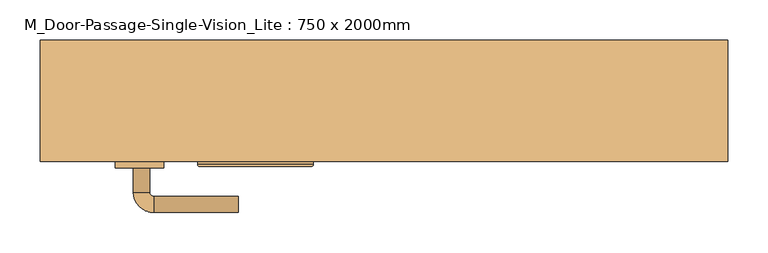
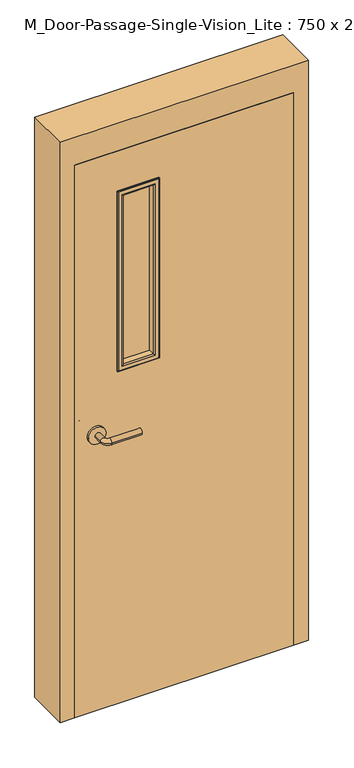
"""IFC4 building model written with IfcOpenShell, lengths in millimetres: door geometry, M_Door-Passage-Single-Vision_Lite : 750 x 2000mm."""

from ifc_helpers import new_model, si_unit, point, frame, frame_2d, origin, place, context, project, spatial, polyline, circle_curve, ellipse_curve, trimmed, segment, composite_curve, outline, extrude, faceted_brep, source, transform, mapped, element, save
from ifc_brep_helpers import plane_surface, cylinder_surface, revolved_surface, advanced_brep


def m_door_passage_single_vision_lite_750_x_2000mm_ab727fbf(model_context):
    return source(origin(), model_context, "Body", "SolidModel", [
        advanced_brep(
        [(-309.990625, 9.15, 1000.0), (-289.990625, 9.15, 1000.0), (-309.990625, 39.15, 1000.0), (-289.990625, 39.15, 1000.0), (-284.990625, 44.15, 1000.0), (-284.990625, 64.15, 1000.0), (-179.990625, 64.15, 1000.0), (-179.990625, 44.15, 1000.0)],
        [
            (0, 1, circle_curve(frame((-299.990625, 9.15, 1000.0), z_axis=(0.0, -1.0, 0.0), x_axis=(1.0, 0.0, 0.0)), 10.0)),
            (1, 0, circle_curve(frame((-299.990625, 9.15, 1000.0), z_axis=(0.0, -1.0, 0.0), x_axis=(1.0, 0.0, 0.0)), 10.0)),
            (0, 2),
            (2, 3, circle_curve(frame((-299.990625, 39.15, 1000.0), z_axis=(0.0, -1.0, 0.0), x_axis=(1.0, 0.0, 0.0)), 10.0)),
            (3, 1),
            (3, 2, circle_curve(frame((-299.990625, 39.15, 1000.0), z_axis=(0.0, -1.0, 0.0), x_axis=(1.0, 0.0, 0.0)), 10.0)),
            (4, 3, circle_curve(frame((-284.990625, 39.15, 1000.0), z_axis=(0.0, 0.0, 1.0), x_axis=(-1.0, 0.0, 0.0)), 5.0)),
            (2, 5, circle_curve(frame((-284.990625, 39.15, 1000.0), z_axis=(0.0, 0.0, -1.0), x_axis=(-1.0, 0.0, 0.0)), 25.0)),
            (5, 4, circle_curve(frame((-284.990625, 54.15, 1000.0), z_axis=(-1.0, 0.0, 0.0), x_axis=(0.0, -1.0, 0.0)), 10.0)),
            (4, 5, circle_curve(frame((-284.990625, 54.15, 1000.0), z_axis=(-1.0, 0.0, 0.0), x_axis=(0.0, -1.0, 0.0)), 10.0)),
            (6, 7, circle_curve(frame((-179.990625, 54.15, 1000.0), z_axis=(1.0, 0.0, 0.0), x_axis=(0.0, -1.0, 0.0)), 10.0)),
            (7, 6, circle_curve(frame((-179.990625, 54.15, 1000.0), z_axis=(1.0, 0.0, 0.0), x_axis=(0.0, -1.0, 0.0)), 10.0)),
            (5, 6),
            (7, 4),
        ],
        [
            plane_surface(frame((-299.990625, 9.15, 1000.0), z_axis=(0.0, -1.0, 0.0), x_axis=(0.0, 0.0, 1.0))),
            cylinder_surface(frame((-299.990625, 9.15, 1000.0), z_axis=(0.0, -1.0, 0.0), x_axis=(1.0, 0.0, 0.0)), 10.0),
            revolved_surface(trimmed(ellipse_curve(frame((-299.990625, 39.15, 1000.0), z_axis=(0.0, -1.0, 0.0), x_axis=(1.0, 0.0, 0.0)), 10.0, 10.0), [point((-309.990625, 39.15, 1000.0))], [point((-289.990625, 39.15, 1000.0))], True, "CARTESIAN"), (-284.990625, 39.15, 1000.0), (0.0, 0.0, -1.0)),
            revolved_surface(trimmed(ellipse_curve(frame((-299.990625, 39.15, 1000.0), z_axis=(0.0, -1.0, 0.0), x_axis=(1.0, 0.0, 0.0)), 10.0, 10.0), [point((-289.990625, 39.15, 1000.0))], [point((-309.990625, 39.15, 1000.0))], True, "CARTESIAN"), (-284.990625, 39.15, 1000.0), (0.0, 0.0, -1.0)),
            plane_surface(frame((-179.990625, 54.15, 1000.0), z_axis=(1.0, 0.0, 0.0), x_axis=(0.0, 0.0, 1.0))),
            cylinder_surface(frame((-284.990625, 54.15, 1000.0), z_axis=(-1.0, 0.0, 0.0), x_axis=(0.0, -1.0, 0.0)), 10.0),
        ],
        [
            (0, [[1, 2]]),
            (1, [[-1, 3, 4, 5]]),
            (1, [[-2, -5, 6, -3]]),
            (2, [[7, -4, 8, 9]]),
            (3, [[-8, -6, -7, 10]]),
            (4, [[11, 12]]),
            (5, [[-9, 13, -12, 14]]),
            (5, [[-10, -14, -11, -13]]),
        ],
    ),
        extrude(outline(composite_curve([segment(trimmed(circle_curve(frame_2d((1000.0, -302.490625)), 30.0), [point((1000.0, -332.490625))], [point((1000.0, -272.490625))], False, "CARTESIAN"), True, "CONTINUOUS"), segment(trimmed(circle_curve(frame_2d((1000.0, -302.490625)), 30.0), [point((1000.0, -272.490625))], [point((1000.0, -332.490625))], False, "CARTESIAN"), True, "CONTINUOUS")], self_intersect=False)), frame((0.0, 1.15, 0.0), z_axis=(0.0, 1.0, 0.0), x_axis=(0.0, 0.0, 1.0)), (0.0, 0.0, 1.0), 8.0),
        advanced_brep(
        [(-309.990625, -51.85, 1000.0), (-289.990625, -51.85, 1000.0), (-289.990625, -81.85, 1000.0), (-309.990625, -81.85, 1000.0), (-284.990625, -86.85, 1000.0), (-284.990625, -106.85, 1000.0), (-179.990625, -106.85, 1000.0), (-179.990625, -86.85, 1000.0)],
        [
            (0, 1, circle_curve(frame((-299.990625, -51.85, 1000.0), z_axis=(0.0, 1.0, 0.0), x_axis=(1.0, 0.0, 0.0)), 10.0)),
            (1, 0, circle_curve(frame((-299.990625, -51.85, 1000.0), z_axis=(0.0, 1.0, 0.0), x_axis=(1.0, 0.0, 0.0)), 10.0)),
            (1, 2),
            (2, 3, circle_curve(frame((-299.990625, -81.85, 1000.0), z_axis=(0.0, 1.0, 0.0), x_axis=(1.0, 0.0, 0.0)), 10.0)),
            (3, 0),
            (3, 2, circle_curve(frame((-299.990625, -81.85, 1000.0), z_axis=(0.0, 1.0, 0.0), x_axis=(1.0, 0.0, 0.0)), 10.0)),
            (4, 5, circle_curve(frame((-284.990625, -96.85, 1000.0), z_axis=(-1.0, 0.0, 0.0), x_axis=(0.0, 1.0, 0.0)), 10.0)),
            (5, 3, circle_curve(frame((-284.990625, -81.85, 1000.0), z_axis=(0.0, 0.0, -1.0), x_axis=(-1.0, 0.0, 0.0)), 25.0)),
            (2, 4, circle_curve(frame((-284.990625, -81.85, 1000.0), z_axis=(0.0, 0.0, 1.0), x_axis=(-1.0, 0.0, 0.0)), 5.0)),
            (5, 4, circle_curve(frame((-284.990625, -96.85, 1000.0), z_axis=(-1.0, 0.0, 0.0), x_axis=(0.0, 1.0, 0.0)), 10.0)),
            (6, 7, circle_curve(frame((-179.990625, -96.85, 1000.0), z_axis=(1.0, 0.0, 0.0), x_axis=(0.0, 1.0, 0.0)), 10.0)),
            (7, 6, circle_curve(frame((-179.990625, -96.85, 1000.0), z_axis=(1.0, 0.0, 0.0), x_axis=(0.0, 1.0, 0.0)), 10.0)),
            (4, 7),
            (6, 5),
        ],
        [
            plane_surface(frame((-299.990625, -51.85, 1000.0), z_axis=(0.0, 1.0, 0.0), x_axis=(0.0, 0.0, 1.0))),
            cylinder_surface(frame((-299.990625, -51.85, 1000.0), z_axis=(0.0, 1.0, 0.0), x_axis=(1.0, 0.0, 0.0)), 10.0),
            revolved_surface(trimmed(ellipse_curve(frame((-299.990625, -81.85, 1000.0), z_axis=(0.0, -1.0, 0.0), x_axis=(1.0, 0.0, 0.0)), 10.0, 10.0), [point((-309.990625, -81.85, 1000.0))], [point((-289.990625, -81.85, 1000.0))], True, "CARTESIAN"), (-284.990625, -81.85, 1000.0), (0.0, 0.0, -1.0)),
            revolved_surface(trimmed(ellipse_curve(frame((-299.990625, -81.85, 1000.0), z_axis=(0.0, -1.0, 0.0), x_axis=(1.0, 0.0, 0.0)), 10.0, 10.0), [point((-289.990625, -81.85, 1000.0))], [point((-309.990625, -81.85, 1000.0))], True, "CARTESIAN"), (-284.990625, -81.85, 1000.0), (0.0, 0.0, -1.0)),
            plane_surface(frame((-179.990625, -96.85, 1000.0), z_axis=(1.0, 0.0, 0.0), x_axis=(0.0, 0.0, 1.0))),
            cylinder_surface(frame((-284.990625, -96.85, 1000.0), z_axis=(-1.0, 0.0, 0.0), x_axis=(0.0, 1.0, 0.0)), 10.0),
        ],
        [
            (0, [[1, 2]]),
            (1, [[3, 4, 5, -2]]),
            (1, [[-5, 6, -3, -1]]),
            (2, [[7, 8, -4, 9]]),
            (3, [[10, -9, -6, -8]]),
            (4, [[11, 12]]),
            (5, [[13, -11, 14, -7]]),
            (5, [[-14, -12, -13, -10]]),
        ],
    ),
        extrude(outline(composite_curve([segment(trimmed(circle_curve(frame_2d((1000.0, -302.490625)), 30.0), [point((1000.0, -332.490625))], [point((1000.0, -272.490625))], False, "CARTESIAN"), True, "CONTINUOUS"), segment(trimmed(circle_curve(frame_2d((1000.0, -302.490625)), 30.0), [point((1000.0, -272.490625))], [point((1000.0, -332.490625))], False, "CARTESIAN"), True, "CONTINUOUS")], self_intersect=False)), frame((0.0, -51.85, 0.0), z_axis=(0.0, 1.0, 0.0), x_axis=(0.0, 0.0, 1.0)), (0.0, 0.0, 1.0), 8.0),
        extrude(outline(polyline([(2000.0, -375.0), (0.0, -375.0), (0.0, 375.0), (2000.0, 375.0), (2000.0, -375.0)]), holes=[polyline([(1847.6, -222.6), (1847.6, -95.6), (1212.6, -95.6), (1212.6, -222.6), (1847.6, -222.6)])]), frame((0.0, -43.85, 0.0), z_axis=(0.0, 1.0, 0.0), x_axis=(0.0, 0.0, 1.0)), (0.0, 0.0, 1.0), 45.0),
        faceted_brep([(375.0, 5.9125, 0.0), (359.125, 5.9125, 0.0), (359.125, 56.9375, 0.0), (375.0, 56.9375, 0.0), (375.0, 106.15, 0.0), (425.0, 106.15, 0.0), (425.0, -43.85, 0.0), (375.0, -43.85, 0.0), (375.0, -43.85, 2000.0), (375.0, 5.9125, 2000.0), (425.0, -43.85, 2100.0), (-425.0, -43.85, 2100.0), (-425.0, -43.85, 0.0), (-375.0, -43.85, 0.0), (-375.0, -43.85, 2000.0), (425.0, 106.15, 2100.0), (375.0, 106.15, 2000.0), (-375.0, 106.15, 2000.0), (-375.0, 106.15, 0.0), (-425.0, 106.15, 0.0), (-425.0, 106.15, 2100.0), (375.0, 56.9375, 2000.0), (359.125, 56.9375, 1984.125), (-359.125, 56.9375, 1984.125), (-359.125, 56.9375, 0.0), (-375.0, 56.9375, 0.0), (-375.0, 56.9375, 2000.0), (359.125, 5.9125, 1984.125), (-375.0, 5.9125, 2000.0), (-375.0, 5.9125, 0.0), (-359.125, 5.9125, 0.0), (-359.125, 5.9125, 1984.125)], [[[0, 1, 2, 3, 4, 5, 6, 7]], [[7, 8, 9, 0]], [[6, 10, 11, 12, 13, 14, 8, 7]], [[5, 15, 10, 6]], [[4, 16, 17, 18, 19, 20, 15, 5]], [[3, 21, 16, 4]], [[2, 22, 23, 24, 25, 26, 21, 3]], [[1, 27, 22, 2]], [[0, 9, 28, 29, 30, 31, 27, 1]], [[8, 14, 28, 9]], [[16, 21, 26, 17]], [[22, 27, 31, 23]], [[12, 19, 18, 25, 24, 30, 29, 13]], [[13, 29, 28, 14]], [[11, 20, 19, 12]], [[17, 26, 25, 18]], [[23, 31, 30, 24]], [[15, 20, 11, 10]]]),
        extrude(outline(polyline([(-95.6, -18.85), (-95.6, -23.85), (-222.6, -23.85), (-222.6, -18.85), (-95.6, -18.85)])), frame((0.0, 0.0, 1212.6), z_axis=(0.0, 0.0, 1.0), x_axis=(1.0, 0.0, 0.0)), (0.0, 0.0, 1.0), 635.0),
        advanced_brep(
        [(-222.6, -23.85, 1847.6), (-222.6, -23.85, 1212.6), (-222.6, -43.85, 1212.6), (-222.6, -43.85, 1847.6), (-210.6, -44.85, 1835.6), (-210.6, -44.85, 1224.6), (-210.6, -23.85, 1224.6), (-210.6, -23.85, 1835.6), (-215.6, -49.85, 1840.6), (-215.6, -49.85, 1219.6), (-230.6, -47.85, 1855.6), (-230.6, -47.85, 1204.6), (-228.6, -49.85, 1206.6), (-228.6, -49.85, 1853.6), (-230.6, -43.85, 1855.6), (-230.6, -43.85, 1204.6), (-95.6, -23.85, 1212.6), (-95.6, -43.85, 1212.6), (-107.6, -44.85, 1224.6), (-107.6, -23.85, 1224.6), (-102.6, -49.85, 1219.6), (-87.6, -47.85, 1204.6), (-89.6, -49.85, 1206.6), (-87.6, -43.85, 1204.6), (-95.6, -23.85, 1847.6), (-95.6, -43.85, 1847.6), (-107.6, -44.85, 1835.6), (-107.6, -23.85, 1835.6), (-102.6, -49.85, 1840.6), (-87.6, -47.85, 1855.6), (-89.6, -49.85, 1853.6), (-87.6, -43.85, 1855.6)],
        [
            (0, 1),
            (1, 2),
            (2, 3),
            (3, 0),
            (4, 5),
            (5, 6),
            (6, 7),
            (7, 4),
            (8, 9),
            (9, 5, ellipse_curve(frame((-215.6, -44.85, 1219.6), z_axis=(-0.7071067811865475, 0.0, 0.7071067811865475), x_axis=(0.7071067811865474, 0.0, 0.7071067811865476)), 7.0710678, 5.0)),
            (4, 8, ellipse_curve(frame((-215.6, -44.85, 1840.6), z_axis=(-0.7071067811865475, 0.0, -0.7071067811865475), x_axis=(-0.7071067811865474, 0.0, 0.7071067811865476)), 7.0710678, 5.0)),
            (10, 11),
            (11, 12, ellipse_curve(frame((-228.6, -47.85, 1206.6), z_axis=(-0.7071067811865475, 0.0, 0.7071067811865475), x_axis=(0.7071067811865474, 0.0, 0.7071067811865476)), 2.8284271, 2.0)),
            (12, 13),
            (13, 10, ellipse_curve(frame((-228.6, -47.85, 1853.6), z_axis=(-0.7071067811865475, 0.0, -0.7071067811865475), x_axis=(-0.7071067811865474, 0.0, 0.7071067811865476)), 2.8284271, 2.0)),
            (14, 15),
            (15, 11),
            (10, 14),
            (1, 16),
            (16, 17),
            (17, 2),
            (5, 18),
            (18, 19),
            (19, 6),
            (9, 20),
            (20, 18, ellipse_curve(frame((-102.6, -44.85, 1219.6), z_axis=(-0.7071067811865475, 0.0, -0.7071067811865475), x_axis=(-0.7071067811865476, 0.0, 0.7071067811865474)), 7.0710678, 5.0)),
            (11, 21),
            (21, 22, ellipse_curve(frame((-89.6, -47.85, 1206.6), z_axis=(-0.7071067811865475, 0.0, -0.7071067811865475), x_axis=(-0.7071067811865476, 0.0, 0.7071067811865474)), 2.8284271, 2.0)),
            (22, 12),
            (15, 23),
            (23, 21),
            (16, 24),
            (24, 25),
            (25, 17),
            (18, 26),
            (26, 27),
            (27, 19),
            (20, 28),
            (28, 26, ellipse_curve(frame((-102.6, -44.85, 1840.6), z_axis=(0.7071067811865475, 0.0, -0.7071067811865475), x_axis=(-0.7071067811865474, 0.0, -0.7071067811865476)), 7.0710678, 5.0)),
            (21, 29),
            (29, 30, ellipse_curve(frame((-89.6, -47.85, 1853.6), z_axis=(0.7071067811865475, 0.0, -0.7071067811865475), x_axis=(-0.7071067811865474, 0.0, -0.7071067811865476)), 2.8284271, 2.0)),
            (30, 22),
            (23, 31),
            (31, 29),
            (14, 31),
            (25, 3),
            (24, 0),
            (27, 7),
            (26, 4),
            (28, 8),
            (30, 13),
            (29, 10),
        ],
        [
            plane_surface(frame((-222.6, -43.85, 1847.6), z_axis=(-1.0, 0.0, 0.0), x_axis=(0.0, 0.0, -1.0))),
            plane_surface(frame((-210.6, -23.85, 1835.6), z_axis=(1.0, 0.0, 0.0), x_axis=(0.0, 0.0, -1.0))),
            cylinder_surface(frame((-215.6, -44.85, 1847.6), z_axis=(0.0, 0.0, 1.0), x_axis=(-1.0, 0.0, 0.0)), 5.0),
            cylinder_surface(frame((-228.6, -47.85, 1847.6), z_axis=(0.0, 0.0, 1.0), x_axis=(-1.0, 0.0, 0.0)), 2.0),
            plane_surface(frame((-230.6, -47.85, 1855.6), z_axis=(-1.0, 0.0, 0.0), x_axis=(0.0, 0.0, -1.0))),
            plane_surface(frame((-222.6, -43.85, 1212.6), z_axis=(0.0, 0.0, -1.0), x_axis=(1.0, 0.0, 0.0))),
            plane_surface(frame((-210.6, -23.85, 1224.6), z_axis=(0.0, 0.0, 1.0), x_axis=(1.0, 0.0, 0.0))),
            cylinder_surface(frame((-222.6, -44.85, 1219.6), z_axis=(-1.0, 0.0, 0.0), x_axis=(0.0, 0.0, -1.0)), 5.0),
            cylinder_surface(frame((-222.6, -47.85, 1206.6), z_axis=(-1.0, 0.0, 0.0), x_axis=(0.0, 0.0, -1.0)), 2.0),
            plane_surface(frame((-230.6, -47.85, 1204.6), z_axis=(0.0, 0.0, -1.0), x_axis=(1.0, 0.0, 0.0))),
            plane_surface(frame((-95.6, -43.85, 1212.6), z_axis=(1.0, 0.0, 0.0), x_axis=(0.0, 0.0, 1.0))),
            plane_surface(frame((-107.6, -23.85, 1224.6), z_axis=(-1.0, 0.0, 0.0), x_axis=(0.0, 0.0, 1.0))),
            cylinder_surface(frame((-102.6, -44.85, 1212.6), z_axis=(0.0, 0.0, -1.0), x_axis=(1.0, 0.0, 0.0)), 5.0),
            cylinder_surface(frame((-89.6, -47.85, 1212.6), z_axis=(0.0, 0.0, -1.0), x_axis=(1.0, 0.0, 0.0)), 2.0),
            plane_surface(frame((-87.6, -47.85, 1204.6), z_axis=(1.0, 0.0, 0.0), x_axis=(0.0, 0.0, 1.0))),
            plane_surface(frame((-87.6, -43.85, 1855.6), z_axis=(0.0, 1.0, 0.0), x_axis=(-1.0, 0.0, 0.0))),
            plane_surface(frame((-95.6, -43.85, 1847.6), z_axis=(0.0, 0.0, 1.0), x_axis=(-1.0, 0.0, 0.0))),
            plane_surface(frame((-95.6, -23.85, 1847.6), z_axis=(0.0, 1.0, 0.0), x_axis=(-1.0, 0.0, 0.0))),
            plane_surface(frame((-107.6, -23.85, 1835.6), z_axis=(0.0, 0.0, -1.0), x_axis=(-1.0, 0.0, 0.0))),
            cylinder_surface(frame((-95.6, -44.85, 1840.6), z_axis=(1.0, 0.0, 0.0), x_axis=(0.0, 0.0, 1.0)), 5.0),
            plane_surface(frame((-102.6, -49.85, 1840.6), z_axis=(0.0, -1.0, 0.0), x_axis=(-1.0, 0.0, 0.0))),
            cylinder_surface(frame((-95.6, -47.85, 1853.6), z_axis=(1.0, 0.0, 0.0), x_axis=(0.0, 0.0, 1.0)), 2.0),
            plane_surface(frame((-87.6, -47.85, 1855.6), z_axis=(0.0, 0.0, 1.0), x_axis=(-1.0, 0.0, 0.0))),
        ],
        [
            (0, [[1, 2, 3, 4]]),
            (1, [[5, 6, 7, 8]]),
            (2, [[9, 10, -5, 11]]),
            (3, [[12, 13, 14, 15]]),
            (4, [[16, 17, -12, 18]]),
            (5, [[19, 20, 21, -2]]),
            (6, [[22, 23, 24, -6]]),
            (7, [[25, 26, -22, -10]]),
            (8, [[27, 28, 29, -13]]),
            (9, [[30, 31, -27, -17]]),
            (10, [[32, 33, 34, -20]]),
            (11, [[35, 36, 37, -23]]),
            (12, [[38, 39, -35, -26]]),
            (13, [[40, 41, 42, -28]]),
            (14, [[43, 44, -40, -31]]),
            (15, [[-16, 45, -43, -30], [-3, -21, -34, 46]]),
            (16, [[47, -4, -46, -33]]),
            (17, [[-1, -47, -32, -19], [-7, -24, -37, 48]]),
            (18, [[49, -8, -48, -36]]),
            (19, [[50, -11, -49, -39]]),
            (20, [[-14, -29, -42, 51], [-9, -50, -38, -25]]),
            (21, [[52, -15, -51, -41]]),
            (22, [[-45, -18, -52, -44]]),
        ],
    ),
        advanced_brep(
        [(-222.6, -18.85, 1212.6), (-222.6, -18.85, 1847.6), (-222.6, 1.15, 1847.6), (-222.6, 1.15, 1212.6), (-210.6, 2.15, 1224.6), (-210.6, 2.15, 1835.6), (-210.6, -18.85, 1835.6), (-210.6, -18.85, 1224.6), (-215.6, 7.15, 1219.6), (-215.6, 7.15, 1840.6), (-230.6, 5.15, 1204.6), (-230.6, 5.15, 1855.6), (-228.6, 7.15, 1853.6), (-228.6, 7.15, 1206.6), (-230.6, 1.15, 1204.6), (-230.6, 1.15, 1855.6), (-95.6, -18.85, 1847.6), (-95.6, 1.15, 1847.6), (-107.6, 2.15, 1835.6), (-107.6, -18.85, 1835.6), (-102.6, 7.15, 1840.6), (-87.6, 5.15, 1855.6), (-89.6, 7.15, 1853.6), (-87.6, 1.15, 1855.6), (-95.6, -18.85, 1212.6), (-95.6, 1.15, 1212.6), (-107.6, 2.15, 1224.6), (-107.6, -18.85, 1224.6), (-102.6, 7.15, 1219.6), (-87.6, 5.15, 1204.6), (-89.6, 7.15, 1206.6), (-87.6, 1.15, 1204.6)],
        [
            (0, 1),
            (1, 2),
            (2, 3),
            (3, 0),
            (4, 5),
            (5, 6),
            (6, 7),
            (7, 4),
            (8, 9),
            (9, 5, ellipse_curve(frame((-215.6, 2.15, 1840.6), z_axis=(-0.7071067811865475, 0.0, -0.7071067811865475), x_axis=(0.7071067811865474, 0.0, -0.7071067811865476)), 7.0710678, 5.0)),
            (4, 8, ellipse_curve(frame((-215.6, 2.15, 1219.6), z_axis=(-0.7071067811865475, 0.0, 0.7071067811865475), x_axis=(-0.7071067811865474, 0.0, -0.7071067811865476)), 7.0710678, 5.0)),
            (10, 11),
            (11, 12, ellipse_curve(frame((-228.6, 5.15, 1853.6), z_axis=(-0.7071067811865475, 0.0, -0.7071067811865475), x_axis=(0.7071067811865474, 0.0, -0.7071067811865476)), 2.8284271, 2.0)),
            (12, 13),
            (13, 10, ellipse_curve(frame((-228.6, 5.15, 1206.6), z_axis=(-0.7071067811865475, 0.0, 0.7071067811865475), x_axis=(-0.7071067811865474, 0.0, -0.7071067811865476)), 2.8284271, 2.0)),
            (14, 15),
            (15, 11),
            (10, 14),
            (1, 16),
            (16, 17),
            (17, 2),
            (5, 18),
            (18, 19),
            (19, 6),
            (9, 20),
            (20, 18, ellipse_curve(frame((-102.6, 2.15, 1840.6), z_axis=(-0.7071067811865475, 0.0, 0.7071067811865475), x_axis=(-0.7071067811865476, 0.0, -0.7071067811865474)), 7.0710678, 5.0)),
            (11, 21),
            (21, 22, ellipse_curve(frame((-89.6, 5.15, 1853.6), z_axis=(-0.7071067811865475, 0.0, 0.7071067811865475), x_axis=(-0.7071067811865476, 0.0, -0.7071067811865474)), 2.8284271, 2.0)),
            (22, 12),
            (15, 23),
            (23, 21),
            (16, 24),
            (24, 25),
            (25, 17),
            (18, 26),
            (26, 27),
            (27, 19),
            (20, 28),
            (28, 26, ellipse_curve(frame((-102.6, 2.15, 1219.6), z_axis=(0.7071067811865475, 0.0, 0.7071067811865475), x_axis=(-0.7071067811865474, 0.0, 0.7071067811865476)), 7.0710678, 5.0)),
            (21, 29),
            (29, 30, ellipse_curve(frame((-89.6, 5.15, 1206.6), z_axis=(0.7071067811865475, 0.0, 0.7071067811865475), x_axis=(-0.7071067811865474, 0.0, 0.7071067811865476)), 2.8284271, 2.0)),
            (30, 22),
            (23, 31),
            (31, 29),
            (14, 31),
            (25, 3),
            (24, 0),
            (27, 7),
            (26, 4),
            (28, 8),
            (30, 13),
            (29, 10),
        ],
        [
            plane_surface(frame((-222.6, 1.15, 1212.6), z_axis=(-1.0, 0.0, 0.0), x_axis=(0.0, 0.0, 1.0))),
            plane_surface(frame((-210.6, -18.85, 1224.6), z_axis=(1.0, 0.0, 0.0), x_axis=(0.0, 0.0, 1.0))),
            cylinder_surface(frame((-215.6, 2.15, 1212.6), z_axis=(0.0, 0.0, -1.0), x_axis=(-1.0, 0.0, 0.0)), 5.0),
            cylinder_surface(frame((-228.6, 5.15, 1212.6), z_axis=(0.0, 0.0, -1.0), x_axis=(-1.0, 0.0, 0.0)), 2.0),
            plane_surface(frame((-230.6, 5.15, 1204.6), z_axis=(-1.0, 0.0, 0.0), x_axis=(0.0, 0.0, 1.0))),
            plane_surface(frame((-222.6, 1.15, 1847.6), z_axis=(0.0, 0.0, 1.0), x_axis=(1.0, 0.0, 0.0))),
            plane_surface(frame((-210.6, -18.85, 1835.6), z_axis=(0.0, 0.0, -1.0), x_axis=(1.0, 0.0, 0.0))),
            cylinder_surface(frame((-222.6, 2.15, 1840.6), z_axis=(-1.0, 0.0, 0.0), x_axis=(0.0, 0.0, 1.0)), 5.0),
            cylinder_surface(frame((-222.6, 5.15, 1853.6), z_axis=(-1.0, 0.0, 0.0), x_axis=(0.0, 0.0, 1.0)), 2.0),
            plane_surface(frame((-230.6, 5.15, 1855.6), z_axis=(0.0, 0.0, 1.0), x_axis=(1.0, 0.0, 0.0))),
            plane_surface(frame((-95.6, 1.15, 1847.6), z_axis=(1.0, 0.0, 0.0), x_axis=(0.0, 0.0, -1.0))),
            plane_surface(frame((-107.6, -18.85, 1835.6), z_axis=(-1.0, 0.0, 0.0), x_axis=(0.0, 0.0, -1.0))),
            cylinder_surface(frame((-102.6, 2.15, 1847.6), z_axis=(0.0, 0.0, 1.0), x_axis=(1.0, 0.0, 0.0)), 5.0),
            cylinder_surface(frame((-89.6, 5.15, 1847.6), z_axis=(0.0, 0.0, 1.0), x_axis=(1.0, 0.0, 0.0)), 2.0),
            plane_surface(frame((-87.6, 5.15, 1855.6), z_axis=(1.0, 0.0, 0.0), x_axis=(0.0, 0.0, -1.0))),
            plane_surface(frame((-87.6, 1.15, 1204.6), z_axis=(0.0, -1.0, 0.0), x_axis=(-1.0, 0.0, 0.0))),
            plane_surface(frame((-95.6, 1.15, 1212.6), z_axis=(0.0, 0.0, -1.0), x_axis=(-1.0, 0.0, 0.0))),
            plane_surface(frame((-95.6, -18.85, 1212.6), z_axis=(0.0, -1.0, 0.0), x_axis=(-1.0, 0.0, 0.0))),
            plane_surface(frame((-107.6, -18.85, 1224.6), z_axis=(0.0, 0.0, 1.0), x_axis=(-1.0, 0.0, 0.0))),
            cylinder_surface(frame((-95.6, 2.15, 1219.6), z_axis=(1.0, 0.0, 0.0), x_axis=(0.0, 0.0, -1.0)), 5.0),
            plane_surface(frame((-102.6, 7.15, 1219.6), z_axis=(0.0, 1.0, 0.0), x_axis=(-1.0, 0.0, 0.0))),
            cylinder_surface(frame((-95.6, 5.15, 1206.6), z_axis=(1.0, 0.0, 0.0), x_axis=(0.0, 0.0, -1.0)), 2.0),
            plane_surface(frame((-87.6, 5.15, 1204.6), z_axis=(0.0, 0.0, -1.0), x_axis=(-1.0, 0.0, 0.0))),
        ],
        [
            (0, [[1, 2, 3, 4]]),
            (1, [[5, 6, 7, 8]]),
            (2, [[9, 10, -5, 11]]),
            (3, [[12, 13, 14, 15]]),
            (4, [[16, 17, -12, 18]]),
            (5, [[19, 20, 21, -2]]),
            (6, [[22, 23, 24, -6]]),
            (7, [[25, 26, -22, -10]]),
            (8, [[27, 28, 29, -13]]),
            (9, [[30, 31, -27, -17]]),
            (10, [[32, 33, 34, -20]]),
            (11, [[35, 36, 37, -23]]),
            (12, [[38, 39, -35, -26]]),
            (13, [[40, 41, 42, -28]]),
            (14, [[43, 44, -40, -31]]),
            (15, [[-16, 45, -43, -30], [-3, -21, -34, 46]]),
            (16, [[47, -4, -46, -33]]),
            (17, [[-1, -47, -32, -19], [-7, -24, -37, 48]]),
            (18, [[49, -8, -48, -36]]),
            (19, [[50, -11, -49, -39]]),
            (20, [[-14, -29, -42, 51], [-9, -50, -38, -25]]),
            (21, [[52, -15, -51, -41]]),
            (22, [[-45, -18, -52, -44]]),
        ],
    ),
    ])


if __name__ == "__main__":
    model = new_model("IFC4")
    model_context = context("Model", 3, world=origin())
    ifc_project = project(units=[si_unit("LENGTHUNIT", "METRE", prefix="MILLI")], contexts=[model_context])
    site = spatial("IfcSite", under=ifc_project)
    building = spatial("IfcBuilding", under=site)
    placement = place(None, origin())
    m_door_passage_single_vision_lite_750_x_2000mm_shape = m_door_passage_single_vision_lite_750_x_2000mm_ab727fbf(model_context)
    element("IfcDoor", 1, ObjectType="M_Door-Passage-Single-Vision_Lite : 750 x 2000mm", at=placement, inside=building, context=model_context, shape_type="MappedRepresentation", body=[
        mapped(m_door_passage_single_vision_lite_750_x_2000mm_shape, transform((0.0, 0.0, 0.0), x_axis=(1.0, 0.0, 0.0), y_axis=(0.0, 1.0, 0.0), z_axis=(0.0, 0.0, 1.0))),
    ])
    save(model, "model.ifc")

# Revit data of these elements
# Type "M_Door-Passage-Single-Vision_Lite : 750 x 2000mm"
#   Type Mark = "42"
#   Assembly Code = "B2030100"
#   Analytic Construction = "Wooden"
#   Thickness = 45 mm
#   Thermal Resistance (R) = 0.455703 (m²·K)/W
#   Swing Angle [instance default] = 90.00°
#   Strike Height = 1000 mm
#   Rough Width [instance default] = 850 mm
#   Rough Height [instance default] = 2100 mm
#   MFOpeningHeight [instance default] = 100 mm
#   MFOpeningWidth [instance default] = 100 mm
#   Inset Calculate [instance default] = 105 mm
#   Masonry Inset [instance default] = 25 mm
#   Height = 2000 mm
#   Width = 750 mm
#   Heat Transfer Coefficient (U) = 2.19465 W/(m²·K)
#   Masonry Frame Depth = 150 mm
#   Masonry Frame [instance default] = yes
#   Function = 1
#   Dry Wall Frame [instance default] = no
#   Panel Material = Wood - Birch
#   Glazing = Glass
#   Glass Stop Material = Metal - Paint Finish - Grey
#   Frame Material = Metal - Paint Finish - Grey
#   Door Handle Material = Aluminum
#   Visual Light Transmittance = 0
#   Solar Heat Gain Coefficient = 0
#   Wall Closure = (empty or 0)
# Element 1 (IfcDoor, "M_Door-Passage-Single-Vision_Lite : 750 x 2000mm")
#   Materials on its faces: "Metal - Paint Finish - Grey", "Aluminum", "Wood - Birch", "Glass"
# Materials
#   "Wood - Birch": class "Wood", colour RGB 173 132 96, transparency 0, Cost = 0
#   "Glass": class "Glass", colour RGB 245 245 243, transparency 1, Description = "Soda Lime Glass", Cost = 0
#   "Metal - Paint Finish - Grey": class "Paint", colour RGB 178 178 178, transparency 0, Cost = 0
#   "Aluminum": class "Metal", colour RGB 244 245 246, transparency 0, Description = "Aluminum 6061", Cost = 0
